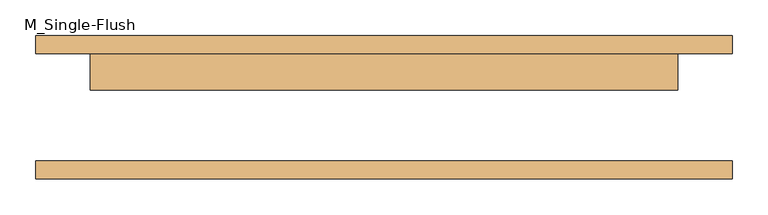
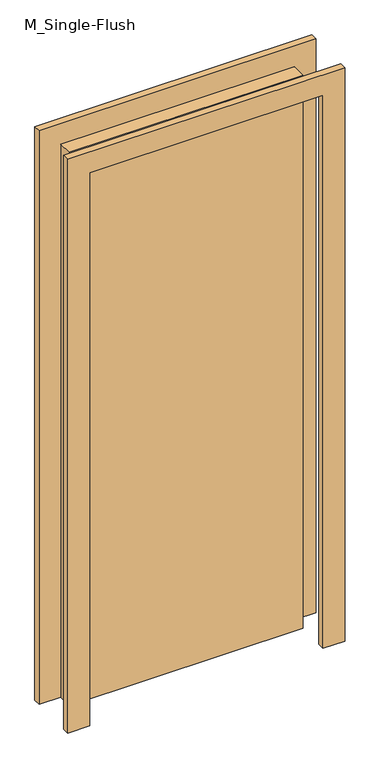
"""IFC4 building model written with IfcOpenShell, lengths in millimetres: door geometry, M_Single-Flush : iç kapı 1."""

import ifcopenshell
import ifcopenshell.guid

model = None  # the IFC model being written
_history = None  # IfcOwnerHistory: only IFC2X3 demands one
_inside = {}  # id of a spatial element -> (the spatial element, [elements in it])
_under = {}  # id of a project, library or spatial element -> (it, [spatial elements below it])
_declared = {}  # id of a project -> (the project, [libraries it declares])
_typed = {}  # id of a type object -> (the type object, [elements of that type])
_made_of = {}  # id of a material, layer set ... -> (it, [elements and type objects made of it])


def new_model(schema):
    """Start an empty IFC model of exactly this schema.

    Asked for "IFC4X3", IfcOpenShell would pick the latest addendum, in which some entities
    have other attributes; the version numbers below select the first issue.
    IFC2X3 requires an IfcOwnerHistory on every rooted entity: one is made here for all.
    """
    global model, _history
    if schema == "IFC4X3":
        model = ifcopenshell.file(schema_version=(4, 3, 0, 0))
    else:
        model = ifcopenshell.file(schema=schema)
    _inside.clear()
    _under.clear()
    _declared.clear()
    _typed.clear()
    _made_of.clear()
    _history = None
    if model.schema == "IFC2X3":
        org = make("IfcOrganization", Name="unknown")
        user = make(
            "IfcPersonAndOrganization",
            ThePerson=make("IfcPerson", FamilyName="unknown"),
            TheOrganization=org,
        )
        app = make(
            "IfcApplication",
            ApplicationDeveloper=org,
            Version="unknown",
            ApplicationFullName="unknown",
            ApplicationIdentifier="unknown",
        )
        _history = make(
            "IfcOwnerHistory",
            OwningUser=user,
            OwningApplication=app,
            ChangeAction="ADDED",
            CreationDate=0,
        )
    return model


def make(cls, **values):
    """One entity of the class cls with the attributes given. An attribute that is None is left unset."""
    return model.create_entity(
        cls, **{name: value for name, value in values.items() if value is not None}
    )


def rooted(cls, **values):
    """An entity with a GlobalId (a new one), such as an element, a storey or a relation."""
    return make(cls, GlobalId=ifcopenshell.guid.new(), OwnerHistory=_history, **values)


def si_unit(unit_type, name, prefix=None):
    """IfcSIUnit, for example si_unit("LENGTHUNIT", "METRE", prefix="MILLI")."""
    return make("IfcSIUnit", UnitType=unit_type, Prefix=prefix, Name=name)


def assignment(units):
    """IfcUnitAssignment: the units of a project."""
    return None if units is None else make("IfcUnitAssignment", Units=units)


def point(xyz):
    """IfcCartesianPoint."""
    return None if xyz is None else make("IfcCartesianPoint", Coordinates=xyz)


def direction(xyz):
    """IfcDirection."""
    return None if xyz is None else make("IfcDirection", DirectionRatios=xyz)


def frame(location, z_axis=None, x_axis=None):
    """IfcAxis2Placement3D, a coordinate frame: its origin and axes. An axis left out is left unset."""
    return make(
        "IfcAxis2Placement3D",
        Location=point(location),
        Axis=direction(z_axis),
        RefDirection=direction(x_axis),
    )


def origin():
    """The frame at (0, 0, 0) with its axes left unset."""
    return frame((0.0, 0.0, 0.0))


def origin_with_axes():
    """The frame at (0, 0, 0) with the z axis (0, 0, 1) and the x axis (1, 0, 0) written out."""
    return frame((0.0, 0.0, 0.0), z_axis=(0.0, 0.0, 1.0), x_axis=(1.0, 0.0, 0.0))


def place(relative_to, where):
    """IfcLocalPlacement: puts the frame where relative to a parent placement (None: the world)."""
    return make(
        "IfcLocalPlacement", PlacementRelTo=relative_to, RelativePlacement=where
    )


def context(
    kind, dimensions, precision=None, world=None, true_north=None, identifier=None
):
    """IfcGeometricRepresentationContext, for example the 3D "Model" context."""
    return make(
        "IfcGeometricRepresentationContext",
        ContextIdentifier=identifier,
        ContextType=kind,
        CoordinateSpaceDimension=dimensions,
        Precision=precision,
        WorldCoordinateSystem=world,
        TrueNorth=true_north,
    )


def project(units=None, contexts=None):
    """IfcProject with its units and contexts."""
    return rooted(
        "IfcProject",
        Name="project",
        RepresentationContexts=contexts,
        UnitsInContext=assignment(units),
    )


def spatial(cls, under=None, at=None, **own):
    """A site, building, storey or space (cls), placed at a placement, below another one or the project."""
    s = rooted(cls, ObjectPlacement=at, **own)
    if under is not None:
        _under.setdefault(under.id(), (under, []))[1].append(s)
    return s


def polyline(points):
    """IfcPolyline through the points."""
    return make("IfcPolyline", Points=[point(p) for p in points])


def outline(outer, holes=None, kind="AREA"):
    """IfcArbitraryClosedProfileDef: a profile drawn as a closed curve; with holes, ...WithVoids."""
    if holes is None:
        return make("IfcArbitraryClosedProfileDef", ProfileType=kind, OuterCurve=outer)
    return make(
        "IfcArbitraryProfileDefWithVoids",
        ProfileType=kind,
        OuterCurve=outer,
        InnerCurves=holes,
    )


def extrude(swept, where, along, depth):
    """IfcExtrudedAreaSolid: the profile swept, set in the frame where, extruded along a direction by depth."""
    return make(
        "IfcExtrudedAreaSolid",
        SweptArea=swept,
        Position=where,
        ExtrudedDirection=direction(along),
        Depth=depth,
    )


def shape(context_of_items, identifier, shape_type, items):
    """IfcShapeRepresentation: the items that make up one representation, for example the "Body"."""
    return make(
        "IfcShapeRepresentation",
        ContextOfItems=context_of_items,
        RepresentationIdentifier=identifier,
        RepresentationType=shape_type,
        Items=items,
    )


def source(mapping_origin, context_of_items, identifier, shape_type, items):
    """IfcRepresentationMap: a shape defined once, which mapped items show again and again."""
    return make(
        "IfcRepresentationMap",
        MappingOrigin=mapping_origin,
        MappedRepresentation=shape(context_of_items, identifier, shape_type, items),
    )


def transform(
    local_origin,
    x_axis=None,
    y_axis=None,
    z_axis=None,
    scale=None,
    scale2=None,
    scale3=None,
    uniform=True,
):
    """IfcCartesianTransformationOperator3D, or its non-uniform kind. x_axis, y_axis, z_axis: its Axis1, 2, 3."""
    if uniform:
        return make(
            "IfcCartesianTransformationOperator3D",
            Axis1=direction(x_axis),
            Axis2=direction(y_axis),
            LocalOrigin=point(local_origin),
            Scale=scale,
            Axis3=direction(z_axis),
        )
    return make(
        "IfcCartesianTransformationOperator3DnonUniform",
        Axis1=direction(x_axis),
        Axis2=direction(y_axis),
        LocalOrigin=point(local_origin),
        Scale=scale,
        Axis3=direction(z_axis),
        Scale2=scale2,
        Scale3=scale3,
    )


def mapped(mapping_source, mapping_target):
    """IfcMappedItem: shows the shape of a source again, moved by a transform."""
    return make(
        "IfcMappedItem", MappingSource=mapping_source, MappingTarget=mapping_target
    )


def made_of(thing, what):
    """Note that an element or type object is made of a material, layer set ...; save() writes the relation."""
    if what is not None:
        _made_of.setdefault(what.id(), (what, []))[1].append(thing)
    return thing


def element(
    cls,
    number,
    at=None,
    inside=None,
    cuts=None,
    type_object=None,
    material=None,
    context=None,
    identifier="Body",
    shape_type=None,
    held_by="IfcProductDefinitionShape",
    body=None,
    shapes=None,
    **own,
):
    """One element of the class cls, such as IfcWall. Its Tag is "e" and its number.

    at: its placement. inside: the storey or other place that contains it. cuts: it is an
    opening in that element (IfcRelVoidsElement). A single representation is given by context,
    identifier, shape_type and body (its items); several are given by shapes. held_by: the class
    of the entity that holds the representations. save() writes the other relations.
    """
    e = rooted(cls, Tag="e%d" % number, ObjectPlacement=at, **own)
    if body is not None:
        shapes = [shape(context, identifier, shape_type, body)]
    if shapes is not None:
        e.Representation = make(held_by, Representations=shapes)
    if inside is not None:
        _inside.setdefault(inside.id(), (inside, []))[1].append(e)
    if cuts is not None:
        rooted(
            "IfcRelVoidsElement", RelatingBuildingElement=cuts, RelatedOpeningElement=e
        )
    if type_object is not None:
        _typed.setdefault(type_object.id(), (type_object, []))[1].append(e)
    return made_of(e, material)


def aggregate(whole, parts):
    """IfcRelAggregates: a whole, such as a stair, and the parts it consists of."""
    return rooted("IfcRelAggregates", RelatingObject=whole, RelatedObjects=parts)


def save(model, path):
    """Write the relations noted so far, then the file.

    IfcRelAggregates (storeys below a building ...), IfcRelContainedInSpatialStructure (elements
    in a storey), IfcRelDefinesByType, IfcRelAssociatesMaterial and IfcRelDeclares: one each for
    every whole, place, type object, material and project.
    """
    for whole, parts in _under.values():
        aggregate(whole, parts)
    for where, things in _inside.values():
        rooted(
            "IfcRelContainedInSpatialStructure",
            RelatedElements=things,
            RelatingStructure=where,
        )
    for kind, things in _typed.values():
        rooted("IfcRelDefinesByType", RelatedObjects=things, RelatingType=kind)
    for what, things in _made_of.values():
        rooted("IfcRelAssociatesMaterial", RelatedObjects=things, RelatingMaterial=what)
    for by, libraries in _declared.values():
        rooted("IfcRelDeclares", RelatingContext=by, RelatedDefinitions=libraries)
    model.write(path)


def m_single_flush_16974dc2(model_context):
    return source(origin(), model_context, "Body", "SweptSolid", [
        extrude(outline(polyline([(2126.0, -486.0), (0.0, -486.0), (0.0, -410.0), (2050.0, -410.0), (2050.0, 410.0), (0.0, 410.0), (0.0, 486.0), (2126.0, 486.0), (2126.0, -486.0)])), frame((0.0, 75.0, 0.0), z_axis=(0.0, 1.0, 0.0), x_axis=(0.0, 0.0, 1.0)), (0.0, 0.0, 1.0), 25.0),
        extrude(outline(polyline([(2126.0, 486.0), (2126.0, -486.0), (0.0, -486.0), (0.0, -410.0), (2050.0, -410.0), (2050.0, 410.0), (0.0, 410.0), (0.0, 486.0), (2126.0, 486.0)])), frame((0.0, -100.0, 0.0), z_axis=(0.0, 1.0, 0.0), x_axis=(0.0, 0.0, 1.0)), (0.0, 0.0, 1.0), 25.0),
        extrude(outline(polyline([(410.0, 24.0), (-410.0, 24.0), (-410.0, 75.0), (410.0, 75.0), (410.0, 24.0)])), origin_with_axes(), (0.0, 0.0, 1.0), 2050.0),
    ])


if __name__ == "__main__":
    model = new_model("IFC4")
    model_context = context("Model", 3, world=origin())
    ifc_project = project(units=[si_unit("LENGTHUNIT", "METRE", prefix="MILLI")], contexts=[model_context])
    site = spatial("IfcSite", under=ifc_project)
    building = spatial("IfcBuilding", under=site)
    placement = place(None, origin())
    m_single_flush_shape = m_single_flush_16974dc2(model_context)
    element("IfcDoor", 1, ObjectType="M_Single-Flush : iç kapı 1", at=placement, inside=building, context=model_context, shape_type="MappedRepresentation", body=[
        mapped(m_single_flush_shape, transform((0.0, 0.0, 0.0), x_axis=(1.0, 0.0, 0.0), y_axis=(0.0, 1.0, 0.0), z_axis=(0.0, 0.0, 1.0))),
    ])
    save(model, "model.ifc")

# Revit data of these elements
# Type "M_Single-Flush : iç kapı 1"
#   Type Mark = "24"
#   Construction Type Id = "MDOOR"
#   Analytic Construction = "Metal"
#   Thickness = 5.1 cm
#   Thermal Resistance (R) = 0.270117 (m²·K)/W
#   Heat Transfer Coefficient (U) = 3.7021 W/(m²·K)
#   Height = 205 cm
#   Trim Projection Ext = 2.5 cm
#   Trim Projection Int = 2.5 cm
#   Trim Width = 7.6 cm
#   Width = 82 cm
#   Define Thermal Properties by = 1
#   Door Material = Door - Panel
#   Frame Material = Door - Frame
#   Visual Light Transmittance = 0
#   Solar Heat Gain Coefficient = 0
#   Function = (empty or 0)
#   Wall Closure = (empty or 0)
# Element 1 (IfcDoor, "M_Single-Flush : iç kapı 1")
#   Materials on its faces: "Door - Frame", "Door - Panel"
# Materials
#   "Door - Panel": class "Wood", colour RGB 210 159 95, transparency 0, Cost = 0
#   "Door - Frame": class "Miscellaneous", colour RGB 118 70 51, transparency 0, Cost = 0
